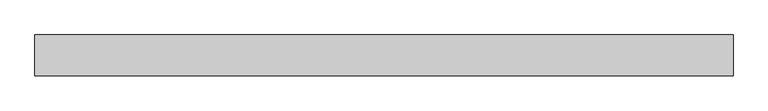
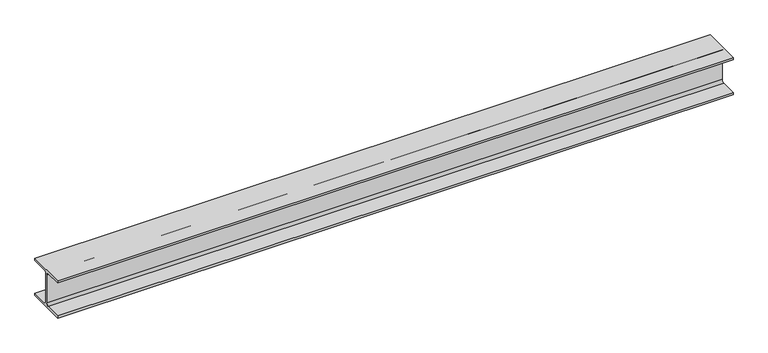
"""IFC4 building model written with IfcOpenShell, lengths in millimetres: beam geometry, 0912_Steel Framing_H-KSD3502 : H_SB_ASB_H-200x200x8x12."""

from ifc_helpers import new_model, si_unit, point, frame, frame_2d, origin, place, context, project, spatial, polyline, circle_curve, trimmed, segment, composite_curve, outline, extrude, source, transform, mapped, element, save


def beam_8fa3f774(model_context):
    return source(origin(), model_context, "Body", "SweptSolid", [
        extrude(outline(composite_curve([segment(polyline([(100.0, -88.0), (100.0, -100.0), (-100.0, -100.0), (-100.0, -88.0), (-17.0, -88.0)]), True, "CONTINUOUS"), segment(trimmed(circle_curve(frame_2d((-17.0, -75.0)), 13.0), [point((-17.0, -88.0))], [point((-4.0, -75.0))], True, "CARTESIAN"), True, "CONTINUOUS"), segment(polyline([(-4.0, -75.0), (-4.0, 75.0)]), True, "CONTINUOUS"), segment(trimmed(circle_curve(frame_2d((-17.0, 75.0)), 13.0), [point((-4.0, 75.0))], [point((-17.0, 88.0))], True, "CARTESIAN"), True, "CONTINUOUS"), segment(polyline([(-17.0, 88.0), (-100.0, 88.0), (-100.0, 100.0), (100.0, 100.0), (100.0, 88.0), (17.0, 88.0)]), True, "CONTINUOUS"), segment(trimmed(circle_curve(frame_2d((17.0, 75.0)), 13.0), [point((17.0, 88.0))], [point((4.0, 75.0))], True, "CARTESIAN"), True, "CONTINUOUS"), segment(polyline([(4.0, 75.0), (4.0, -75.0)]), True, "CONTINUOUS"), segment(trimmed(circle_curve(frame_2d((17.0, -75.0)), 13.0), [point((4.0, -75.0))], [point((17.0, -88.0))], True, "CARTESIAN"), True, "CONTINUOUS"), segment(polyline([(17.0, -88.0), (100.0, -88.0)]), True, "CONTINUOUS")], self_intersect=False)), frame((-1594.6978558, 0.0, 0.0), z_axis=(1.0, 0.0, 0.0), x_axis=(0.0, 1.0, 0.0)), (0.0, 0.0, 1.0), 3419.4191959),
    ])


if __name__ == "__main__":
    model = new_model("IFC4")
    model_context = context("Model", 3, world=origin())
    ifc_project = project(units=[si_unit("LENGTHUNIT", "METRE", prefix="MILLI")], contexts=[model_context])
    site = spatial("IfcSite", under=ifc_project)
    building = spatial("IfcBuilding", under=site)
    placement = place(None, origin())
    beam_shape = beam_8fa3f774(model_context)
    element("IfcBeam", 1, ObjectType="0912_Steel Framing_H-KSD3502 : H_SB_ASB_H-200x200x8x12", at=placement, inside=building, context=model_context, shape_type="MappedRepresentation", body=[
        mapped(beam_shape, transform((0.0, 0.0, 0.0), x_axis=(1.0, 0.0, 0.0), y_axis=(0.0, 1.0, 0.0), z_axis=(0.0, 0.0, 1.0))),
    ])
    save(model, "model.ifc")

# Revit data of these elements
# Type "0912_Steel Framing_H-KSD3502 : H_SB_ASB_H-200x200x8x12"
#   H_WM Code_1 = "S01AA002-00001 | Main Steel Structure Fabrication Work | Shelter/Building | Medium Steel - Standard (90KG/M>Weight≥30KG/M) | Material: (   )"
#   H_WM Code_2 = "S03AA028-00001 | Main Steel Structure Erection Work | Shelter/Building | Medium Steel (90KG/M>Weight≥30KG/M) | Material: (   )"
#   H_WM Code_3 = "S01AA010-00001 | Main Steel Structure Fabrication Work | Shelter/Building | Steel Painting/Coating | for Non-Fireproofed Steel Surface, Surface Preparation, Primer, Second & Final Coat | Material: (   )"
#   H_Q'ty Cal Type Tag = "SB-Q2"
#   Width = 20.0 cm
#   Web Thickness = 0.8 cm
#   Web Fillet = 1.3 cm
#   Warping Constant = 141000.0 cm⁶
#   W = 0
#   Torsional Moment of Inertia = 26.2485 cm⁴
#   Section Area = 63.53 cm²
#   Plastic Modulus weak axis = 244.0 cm³
#   Plastic Modulus strong axis = 525.0 cm³
#   Perimeter = 1.16 m²/m
#   Nominal Weight = 49.90 kgf/m
#   Moment of Inertia weak axis = 1600.00 cm⁴
#   Moment of Inertia strong axis = 4720.00 cm⁴
#   Height = 20.0 cm
#   Flange Thickness = 1.2 cm
#   Elastic Modulus weak axis = 160.0 cm³
#   Elastic Modulus strong axis = 472.0 cm³
#   Centroid Vertical = 10.0 cm
#   Centroid Horizontal = 10.0 cm
#   Ix = 47200000
#   Length [instance default] = 1.5240 m
#   Zx = 525000
#   b = 0.2000 m
#   h = 0.2000 m
#   r = 0.0130 m
#   s = 0.0080 m
#   t = 0.0120 m
#   A = 0.006353 m²
#   Structural Material [instance default] = Steel, 45-345
#   Assembly Code = ""
# Element 1 (IfcBeam, "0912_Steel Framing_H-KSD3502 : H_SB_ASB_H-200x200x8x12")
#   Structural Material = none
# Materials
#   "Steel, 45-345": class "Metal", colour RGB 189 187 185, transparency 0, Description = "Steel 345 MPa", Cost = 0
